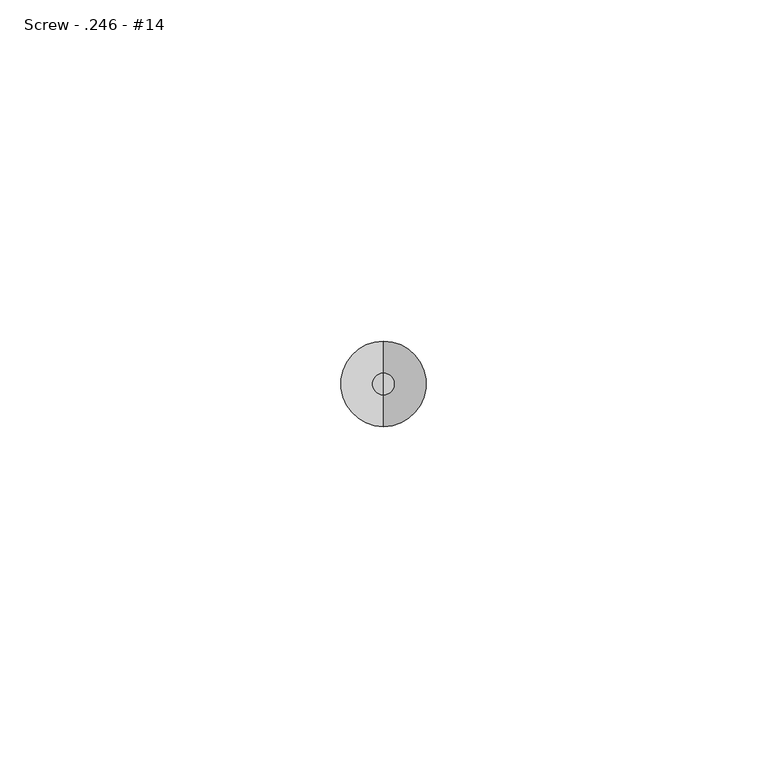
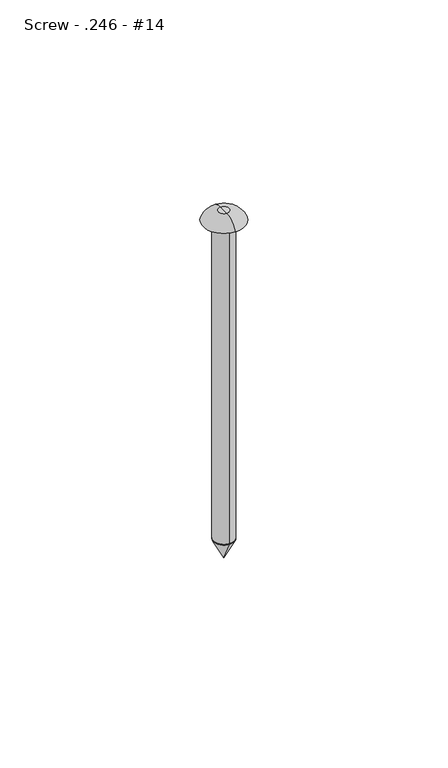
"""IFC4 building model written with IfcOpenShell, lengths in millimetres: fastener geometry, 060523 - W_P_C - Fastenings - Generic : Screw - .246 - #14."""

import ifcopenshell
import ifcopenshell.guid

model = None  # the IFC model being written
_history = None  # IfcOwnerHistory: only IFC2X3 demands one
_inside = {}  # id of a spatial element -> (the spatial element, [elements in it])
_under = {}  # id of a project, library or spatial element -> (it, [spatial elements below it])
_declared = {}  # id of a project -> (the project, [libraries it declares])
_typed = {}  # id of a type object -> (the type object, [elements of that type])
_made_of = {}  # id of a material, layer set ... -> (it, [elements and type objects made of it])


def new_model(schema):
    """Start an empty IFC model of exactly this schema.

    Asked for "IFC4X3", IfcOpenShell would pick the latest addendum, in which some entities
    have other attributes; the version numbers below select the first issue.
    IFC2X3 requires an IfcOwnerHistory on every rooted entity: one is made here for all.
    """
    global model, _history
    if schema == "IFC4X3":
        model = ifcopenshell.file(schema_version=(4, 3, 0, 0))
    else:
        model = ifcopenshell.file(schema=schema)
    _inside.clear()
    _under.clear()
    _declared.clear()
    _typed.clear()
    _made_of.clear()
    _history = None
    if model.schema == "IFC2X3":
        org = make("IfcOrganization", Name="unknown")
        user = make(
            "IfcPersonAndOrganization",
            ThePerson=make("IfcPerson", FamilyName="unknown"),
            TheOrganization=org,
        )
        app = make(
            "IfcApplication",
            ApplicationDeveloper=org,
            Version="unknown",
            ApplicationFullName="unknown",
            ApplicationIdentifier="unknown",
        )
        _history = make(
            "IfcOwnerHistory",
            OwningUser=user,
            OwningApplication=app,
            ChangeAction="ADDED",
            CreationDate=0,
        )
    return model


def make(cls, **values):
    """One entity of the class cls with the attributes given. An attribute that is None is left unset."""
    return model.create_entity(
        cls, **{name: value for name, value in values.items() if value is not None}
    )


def rooted(cls, **values):
    """An entity with a GlobalId (a new one), such as an element, a storey or a relation."""
    return make(cls, GlobalId=ifcopenshell.guid.new(), OwnerHistory=_history, **values)


def si_unit(unit_type, name, prefix=None):
    """IfcSIUnit, for example si_unit("LENGTHUNIT", "METRE", prefix="MILLI")."""
    return make("IfcSIUnit", UnitType=unit_type, Prefix=prefix, Name=name)


def assignment(units):
    """IfcUnitAssignment: the units of a project."""
    return None if units is None else make("IfcUnitAssignment", Units=units)


def point(xyz):
    """IfcCartesianPoint."""
    return None if xyz is None else make("IfcCartesianPoint", Coordinates=xyz)


def direction(xyz):
    """IfcDirection."""
    return None if xyz is None else make("IfcDirection", DirectionRatios=xyz)


def frame(location, z_axis=None, x_axis=None):
    """IfcAxis2Placement3D, a coordinate frame: its origin and axes. An axis left out is left unset."""
    return make(
        "IfcAxis2Placement3D",
        Location=point(location),
        Axis=direction(z_axis),
        RefDirection=direction(x_axis),
    )


def frame_2d(location, x_axis=None):
    """IfcAxis2Placement2D, a coordinate frame in the plane: its origin and x axis."""
    return make(
        "IfcAxis2Placement2D", Location=point(location), RefDirection=direction(x_axis)
    )


def origin():
    """The frame at (0, 0, 0) with its axes left unset."""
    return frame((0.0, 0.0, 0.0))


def origin_2d():
    """The frame at (0, 0) in the plane with its x axis left unset."""
    return frame_2d((0.0, 0.0))


def place(relative_to, where):
    """IfcLocalPlacement: puts the frame where relative to a parent placement (None: the world)."""
    return make(
        "IfcLocalPlacement", PlacementRelTo=relative_to, RelativePlacement=where
    )


def context(
    kind, dimensions, precision=None, world=None, true_north=None, identifier=None
):
    """IfcGeometricRepresentationContext, for example the 3D "Model" context."""
    return make(
        "IfcGeometricRepresentationContext",
        ContextIdentifier=identifier,
        ContextType=kind,
        CoordinateSpaceDimension=dimensions,
        Precision=precision,
        WorldCoordinateSystem=world,
        TrueNorth=true_north,
    )


def project(units=None, contexts=None):
    """IfcProject with its units and contexts."""
    return rooted(
        "IfcProject",
        Name="project",
        RepresentationContexts=contexts,
        UnitsInContext=assignment(units),
    )


def spatial(cls, under=None, at=None, **own):
    """A site, building, storey or space (cls), placed at a placement, below another one or the project."""
    s = rooted(cls, ObjectPlacement=at, **own)
    if under is not None:
        _under.setdefault(under.id(), (under, []))[1].append(s)
    return s


def polyline(points):
    """IfcPolyline through the points."""
    return make("IfcPolyline", Points=[point(p) for p in points])


def circle_curve(where, radius):
    """IfcCircle in the frame where."""
    return make("IfcCircle", Position=where, Radius=radius)


def ellipse_curve(where, semi_axis1, semi_axis2):
    """IfcEllipse in the frame where."""
    return make(
        "IfcEllipse", Position=where, SemiAxis1=semi_axis1, SemiAxis2=semi_axis2
    )


def trimmed(basis, trim1, trim2, sense, master):
    """IfcTrimmedCurve: the piece of a basis curve between two trims."""
    return make(
        "IfcTrimmedCurve",
        BasisCurve=basis,
        Trim1=trim1,
        Trim2=trim2,
        SenseAgreement=sense,
        MasterRepresentation=master,
    )


def segment(curve, same_sense, transition):
    """IfcCompositeCurveSegment."""
    return make(
        "IfcCompositeCurveSegment",
        Transition=transition,
        SameSense=same_sense,
        ParentCurve=curve,
    )


def composite_curve(segments, self_intersect=None):
    """IfcCompositeCurve: segments joined end to end."""
    return make("IfcCompositeCurve", Segments=segments, SelfIntersect=self_intersect)


def outline(outer, holes=None, kind="AREA"):
    """IfcArbitraryClosedProfileDef: a profile drawn as a closed curve; with holes, ...WithVoids."""
    if holes is None:
        return make("IfcArbitraryClosedProfileDef", ProfileType=kind, OuterCurve=outer)
    return make(
        "IfcArbitraryProfileDefWithVoids",
        ProfileType=kind,
        OuterCurve=outer,
        InnerCurves=holes,
    )


def extrude(swept, where, along, depth):
    """IfcExtrudedAreaSolid: the profile swept, set in the frame where, extruded along a direction by depth."""
    return make(
        "IfcExtrudedAreaSolid",
        SweptArea=swept,
        Position=where,
        ExtrudedDirection=direction(along),
        Depth=depth,
    )


def shape(context_of_items, identifier, shape_type, items):
    """IfcShapeRepresentation: the items that make up one representation, for example the "Body"."""
    return make(
        "IfcShapeRepresentation",
        ContextOfItems=context_of_items,
        RepresentationIdentifier=identifier,
        RepresentationType=shape_type,
        Items=items,
    )


def source(mapping_origin, context_of_items, identifier, shape_type, items):
    """IfcRepresentationMap: a shape defined once, which mapped items show again and again."""
    return make(
        "IfcRepresentationMap",
        MappingOrigin=mapping_origin,
        MappedRepresentation=shape(context_of_items, identifier, shape_type, items),
    )


def transform(
    local_origin,
    x_axis=None,
    y_axis=None,
    z_axis=None,
    scale=None,
    scale2=None,
    scale3=None,
    uniform=True,
):
    """IfcCartesianTransformationOperator3D, or its non-uniform kind. x_axis, y_axis, z_axis: its Axis1, 2, 3."""
    if uniform:
        return make(
            "IfcCartesianTransformationOperator3D",
            Axis1=direction(x_axis),
            Axis2=direction(y_axis),
            LocalOrigin=point(local_origin),
            Scale=scale,
            Axis3=direction(z_axis),
        )
    return make(
        "IfcCartesianTransformationOperator3DnonUniform",
        Axis1=direction(x_axis),
        Axis2=direction(y_axis),
        LocalOrigin=point(local_origin),
        Scale=scale,
        Axis3=direction(z_axis),
        Scale2=scale2,
        Scale3=scale3,
    )


def mapped(mapping_source, mapping_target):
    """IfcMappedItem: shows the shape of a source again, moved by a transform."""
    return make(
        "IfcMappedItem", MappingSource=mapping_source, MappingTarget=mapping_target
    )


def made_of(thing, what):
    """Note that an element or type object is made of a material, layer set ...; save() writes the relation."""
    if what is not None:
        _made_of.setdefault(what.id(), (what, []))[1].append(thing)
    return thing


def element(
    cls,
    number,
    at=None,
    inside=None,
    cuts=None,
    type_object=None,
    material=None,
    context=None,
    identifier="Body",
    shape_type=None,
    held_by="IfcProductDefinitionShape",
    body=None,
    shapes=None,
    **own,
):
    """One element of the class cls, such as IfcWall. Its Tag is "e" and its number.

    at: its placement. inside: the storey or other place that contains it. cuts: it is an
    opening in that element (IfcRelVoidsElement). A single representation is given by context,
    identifier, shape_type and body (its items); several are given by shapes. held_by: the class
    of the entity that holds the representations. save() writes the other relations.
    """
    e = rooted(cls, Tag="e%d" % number, ObjectPlacement=at, **own)
    if body is not None:
        shapes = [shape(context, identifier, shape_type, body)]
    if shapes is not None:
        e.Representation = make(held_by, Representations=shapes)
    if inside is not None:
        _inside.setdefault(inside.id(), (inside, []))[1].append(e)
    if cuts is not None:
        rooted(
            "IfcRelVoidsElement", RelatingBuildingElement=cuts, RelatedOpeningElement=e
        )
    if type_object is not None:
        _typed.setdefault(type_object.id(), (type_object, []))[1].append(e)
    return made_of(e, material)


def aggregate(whole, parts):
    """IfcRelAggregates: a whole, such as a stair, and the parts it consists of."""
    return rooted("IfcRelAggregates", RelatingObject=whole, RelatedObjects=parts)


def save(model, path):
    """Write the relations noted so far, then the file.

    IfcRelAggregates (storeys below a building ...), IfcRelContainedInSpatialStructure (elements
    in a storey), IfcRelDefinesByType, IfcRelAssociatesMaterial and IfcRelDeclares: one each for
    every whole, place, type object, material and project.
    """
    for whole, parts in _under.values():
        aggregate(whole, parts)
    for where, things in _inside.values():
        rooted(
            "IfcRelContainedInSpatialStructure",
            RelatedElements=things,
            RelatingStructure=where,
        )
    for kind, things in _typed.values():
        rooted("IfcRelDefinesByType", RelatedObjects=things, RelatingType=kind)
    for what, things in _made_of.values():
        rooted("IfcRelAssociatesMaterial", RelatedObjects=things, RelatingMaterial=what)
    for by, libraries in _declared.values():
        rooted("IfcRelDeclares", RelatingContext=by, RelatedDefinitions=libraries)
    model.write(path)


def plane_surface(at):
    """IfcPlane: the flat surface through the origin of the frame at, square to its z axis."""
    return make("IfcPlane", Position=at)


def revolved_surface(curve, axis_point, axis_direction):
    """IfcSurfaceOfRevolution: the curve turned about the line through axis_point along axis_direction."""
    return make(
        "IfcSurfaceOfRevolution",
        SweptCurve=make("IfcArbitraryOpenProfileDef", ProfileType="CURVE", Curve=curve),
        AxisPosition=make("IfcAxis1Placement", Location=point(axis_point), Axis=direction(axis_direction)),
    )


def advanced_brep(points, edges, surfaces, faces):
    """IfcAdvancedBrep: a solid bounded by faces that lie on surfaces and meet in shared edges.

    An edge is (start, end): straight between two places in points (the first is 0);
    or (start, end, curve); or (start, end, curve, False) where it runs against its curve.
    A face is (place in surfaces, loops), or (place, loops, False) where it looks against
    its surface's normal. A loop lists edges by number (the first is 1), with a minus sign
    where the edge is run from its end to its start. The first loop is the outer one.
    """
    corners = [point(p) for p in points]
    vertices = [make("IfcVertexPoint", VertexGeometry=c) for c in corners]
    made = []
    for start, end, *more in edges:
        made.append(
            make(
                "IfcEdgeCurve",
                EdgeStart=vertices[start],
                EdgeEnd=vertices[end],
                EdgeGeometry=more[0] if more else make("IfcPolyline", Points=[corners[start], corners[end]]),
                SameSense=more[1] if len(more) > 1 else True,
            )
        )
    hull = []
    for where, loops, *sense in faces:
        bounds = []
        for j, loop in enumerate(loops):
            ring = [make("IfcOrientedEdge", EdgeElement=made[abs(k) - 1], Orientation=k > 0) for k in loop]
            bounds.append(
                make(
                    "IfcFaceOuterBound" if j == 0 else "IfcFaceBound",
                    Bound=make("IfcEdgeLoop", EdgeList=ring),
                    Orientation=True,
                )
            )
        hull.append(make("IfcAdvancedFace", Bounds=bounds, FaceSurface=surfaces[where], SameSense=sense[0] if sense else True))
    return make("IfcAdvancedBrep", Outer=make("IfcClosedShell", CfsFaces=hull))


def screw_246_14_ceffc853(model_context):
    return source(origin(), model_context, "Body", "SolidModel", [
        advanced_brep(
        [(0.0, -3.1242, -101.6), (0.0, 3.1242, -101.6), (0.0, 0.0, -101.6), (0.0, 0.0, -107.8484)],
        [
            (0, 1, circle_curve(frame((0.0, 0.0, -101.6), z_axis=(0.0, 0.0, 1.0), x_axis=(0.0, 1.0, 0.0)), 3.1242)),
            (1, 2),
            (2, 0),
            (1, 0, circle_curve(frame((0.0, 0.0, -101.6), z_axis=(0.0, 0.0, 1.0), x_axis=(0.0, 1.0, 0.0)), 3.1242)),
            (3, 1),
            (0, 3),
        ],
        [
            plane_surface(frame((0.0, 0.0, -101.6), z_axis=(0.0, 0.0, 1.0), x_axis=(0.0, 1.0, 0.0))),
            revolved_surface(polyline([(0.0, 3.1242, -101.6), (0.0, 0.0, -107.8484)]), (0.0, 0.0, -103.0840259), (0.0, 0.0, -1.0)),
        ],
        [
            (0, [[1, 2, 3]]),
            (0, [[4, -3, -2]]),
            (1, [[5, -1, 6]]),
            (1, [[-6, -4, -5]]),
        ],
    ),
        advanced_brep(
        [(0.0, 6.2484, 0.0), (0.0, -6.2484, 0.0), (0.0, 0.0, 0.0), (0.0, 0.0, 3.1242), (0.0, -1.5875, 3.1242), (0.0, 1.5875, 3.1242)],
        [
            (0, 1, circle_curve(frame((0.0, 0.0, 0.0), z_axis=(0.0, 0.0, -1.0), x_axis=(0.0, -1.0, 0.0)), 6.2484)),
            (1, 2),
            (2, 0),
            (1, 0, circle_curve(frame((0.0, 0.0, 0.0), z_axis=(0.0, 0.0, -1.0), x_axis=(0.0, -1.0, 0.0)), 6.2484)),
            (3, 4),
            (4, 5, circle_curve(frame((0.0, 0.0, 3.1242), z_axis=(0.0, 0.0, 1.0), x_axis=(0.0, -1.0, 0.0)), 1.5875)),
            (5, 3),
            (5, 4, circle_curve(frame((0.0, 0.0, 3.1242), z_axis=(0.0, 0.0, 1.0), x_axis=(0.0, -1.0, 0.0)), 1.5875)),
            (4, 1, circle_curve(frame((0.0, -1.5875, -1.9146283), z_axis=(1.0, 0.0, 0.0), x_axis=(0.0, -1.0, 0.0)), 5.0388283)),
            (0, 5, circle_curve(frame((0.0, 1.5875, -1.9146283), z_axis=(1.0, 0.0, 0.0), x_axis=(0.0, 1.0, 0.0)), 5.0388283)),
        ],
        [
            plane_surface(frame((0.0, 0.0, 0.0), z_axis=(0.0, 0.0, -1.0), x_axis=(0.0, -1.0, 0.0))),
            plane_surface(frame((0.0, 0.0, 3.1242), z_axis=(0.0, 0.0, 1.0), x_axis=(0.0, -1.0, 0.0))),
            revolved_surface(trimmed(ellipse_curve(frame((0.0, -1.5875, -1.9146283), z_axis=(-1.0, 0.0, 0.0), x_axis=(0.0, -1.0, 0.0)), 5.0388283, 5.0388283), [point((0.0, -6.2484, 0.0))], [point((0.0, -1.5875, 3.1242))], True, "CARTESIAN"), (0.0, 0.0, 1.4840259), (0.0, 0.0, 1.0)),
        ],
        [
            (0, [[1, 2, 3]]),
            (0, [[4, -3, -2]]),
            (1, [[5, 6, 7]]),
            (1, [[-7, 8, -5]]),
            (2, [[-6, 9, -1, 10]]),
            (2, [[-8, -10, -4, -9]]),
        ],
    ),
        extrude(outline(composite_curve([segment(trimmed(circle_curve(origin_2d(), 3.1242), [point((0.0, -3.1242))], [point((0.0, 3.1242))], False, "CARTESIAN"), True, "CONTINUOUS"), segment(trimmed(circle_curve(origin_2d(), 3.1242), [point((0.0, 3.1242))], [point((0.0, -3.1242))], False, "CARTESIAN"), True, "CONTINUOUS")], self_intersect=False)), frame((0.0, 0.0, -101.6), z_axis=(0.0, 0.0, 1.0), x_axis=(1.0, 0.0, 0.0)), (0.0, 0.0, 1.0), 101.6),
    ])


if __name__ == "__main__":
    model = new_model("IFC4")
    model_context = context("Model", 3, world=origin())
    ifc_project = project(units=[si_unit("LENGTHUNIT", "METRE", prefix="MILLI")], contexts=[model_context])
    site = spatial("IfcSite", under=ifc_project)
    building = spatial("IfcBuilding", under=site)
    placement = place(None, origin())
    screw_246_14_shape = screw_246_14_ceffc853(model_context)
    element("IfcFastener", 1, ObjectType="060523 - W_P_C - Fastenings - Generic : Screw - .246 - #14", at=placement, inside=building, context=model_context, shape_type="MappedRepresentation", body=[
        mapped(screw_246_14_shape, transform((0.0, 0.0, 0.0), x_axis=(1.0, 0.0, 0.0), y_axis=(0.0, 1.0, 0.0), z_axis=(0.0, 0.0, 1.0))),
    ])
    save(model, "model.ifc")

# Revit data of these elements
# Type "060523 - W_P_C - Fastenings - Generic : Screw - .246 - #14"
#   Washer_Thickness = 0' - 0.00333"
#   Washer Radius = 0' - 0.133"
#   Washer Offset - Head = 0' - 0"
#   Washer Offset = 0' - 0"
#   Thickness_of_Substrate [instance default] = 0' - 1"
#   Side = 0' - 0 37/64"
#   Radius = 0' - 0.123"
#   Length [instance default] = 0' - 4"
#   Head Size = 0' - 1"
#   Head Radius = 0' - 0 1/2"
#   Head Height = 0' - 0.01"
#   Double Diameter = 0' - 0.492"
#   Diameter = 0' - 0.246"
#   Default Elevation = 4' - 0"
#   Washer_Nut_Visibility = no
#   Washer_Head_Visibility = no
#   Round_Head_Visibility = yes
#   Point Visibility = yes
#   Nut_Visibility = no
#   Hex_Head_Visiblilty = no
#   Washer Material = none
#   Bolt Material (Size) = AT SILL - FASTENER AT 24" O.C.
# Element 1 (IfcFastener, "060523 - W_P_C - Fastenings - Generic : Screw - .246 - #14")
#   Materials on its faces: "AT SILL - FASTENER AT 24\" O.C."
# Materials
#   "AT SILL - FASTENER AT 24\" O.C.": class "Generic", colour RGB 120 120 120, transparency 0, Cost = 0
